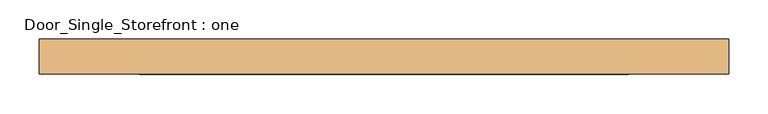
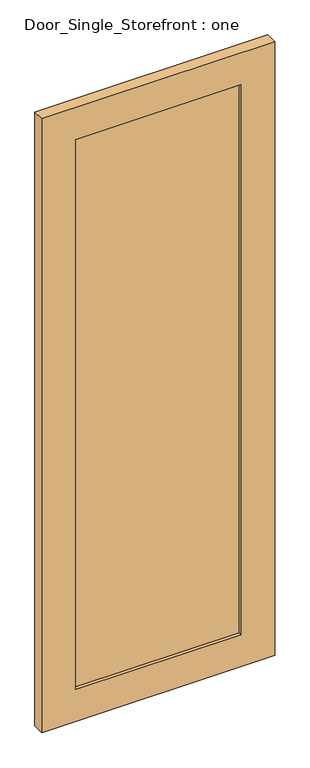
"""IFC4 building model written with IfcOpenShell, lengths in millimetres: door geometry, Door_Single_Storefront : one."""

from ifc_helpers import new_model, si_unit, frame, origin, place, context, project, spatial, polyline, outline, extrude, source, transform, mapped, element, save


def door_single_storefront_one_07ca36dc(model_context):
    return source(origin(), model_context, "Body", "SweptSolid", [
        extrude(outline(polyline([(310.35625, 6.35), (310.35625, -12.7), (-310.35625, -12.7), (-310.35625, 6.35), (310.35625, 6.35)])), frame((0.0, 0.0, 127.0), z_axis=(0.0, 0.0, 1.0), x_axis=(1.0, 0.0, 0.0)), (0.0, 0.0, 1.0), 2184.4),
        extrude(outline(polyline([(2438.4, -437.35625), (0.0, -437.35625), (0.0, 437.35625), (2438.4, 437.35625), (2438.4, -437.35625)]), holes=[polyline([(127.0, 310.35625), (127.0, -310.35625), (2311.4, -310.35625), (2311.4, 310.35625), (127.0, 310.35625)])]), frame((0.0, -25.4, 0.0), z_axis=(0.0, 1.0, 0.0), x_axis=(0.0, 0.0, 1.0)), (0.0, 0.0, 1.0), 44.45),
    ])


if __name__ == "__main__":
    model = new_model("IFC4")
    model_context = context("Model", 3, world=origin())
    ifc_project = project(units=[si_unit("LENGTHUNIT", "METRE", prefix="MILLI")], contexts=[model_context])
    site = spatial("IfcSite", under=ifc_project)
    building = spatial("IfcBuilding", under=site)
    placement = place(None, origin())
    door_single_storefront_one_shape = door_single_storefront_one_07ca36dc(model_context)
    element("IfcDoor", 1, ObjectType="Door_Single_Storefront : one", at=placement, inside=building, context=model_context, shape_type="MappedRepresentation", body=[
        mapped(door_single_storefront_one_shape, transform((0.0, 0.0, 0.0), x_axis=(1.0, 0.0, 0.0), y_axis=(0.0, 1.0, 0.0), z_axis=(0.0, 0.0, 1.0))),
    ])
    save(model, "model.ifc")

# Revit data of these elements
# Type "Door_Single_Storefront : one"
#   Type Mark = "27"
#   Analytic Construction = "<None>"
#   Stile_Width = 0' - 5"
#   Door_Thickness = 0' - 1 3/4"
#   Door_Offset = 0' - 1"
#   Glass_Material = SAFETY GLAZING
#   Frame_Material = INTERIOR GRADE ALUMINUM STOREFRONT W/ SAFETY GLAZING
#   Function = (empty or 0)
# Element 1 (IfcDoor, "Door_Single_Storefront : one")
#   Materials on its faces: "INTERIOR GRADE ALUMINUM STOREFRONT W/ SAFETY GLAZING", "SAFETY GLAZING"
# Materials
#   "SAFETY GLAZING": class "Glass", colour RGB 142 168 196, transparency 0.75, Description = "Soda Lime Glass", Cost = 0
#   "INTERIOR GRADE ALUMINUM STOREFRONT W/ SAFETY GLAZING": class "Metal", colour RGB 226 226 226, transparency 0, Description = "Aluminum 6061", Cost = 0
